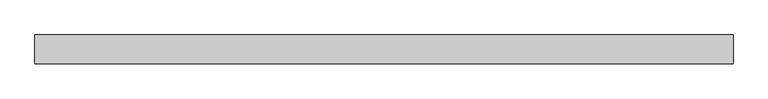
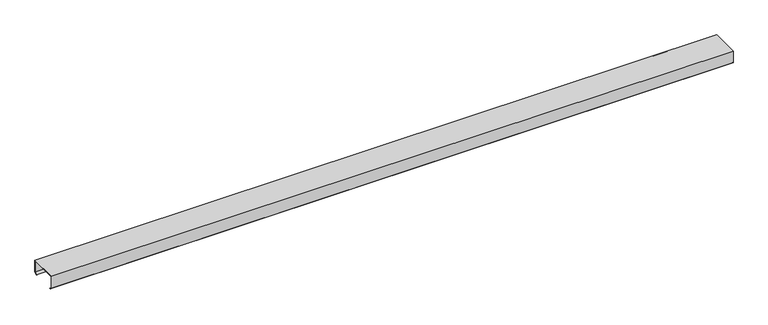
"""IFC4 building model written with IfcOpenShell, lengths in millimetres: proxy geometry, Generic Models 7:Generic Models 1:1:Generic Models 1:1 : Generic Models 7:Generic Models 1:337419:20 : Generic Models 7:Generic Models 1:1:Generic Models 1:1 : Generic Models 7:Generic Models 1:337419:306201."""

from ifc_helpers import new_model, si_unit, frame, origin, place, context, project, spatial, polyline, outline, extrude, source, transform, mapped, element, save


def generic_models_f52606a6(model_context):
    return source(origin(), model_context, "Body", "SweptSolid", [
        extrude(outline(polyline([(-578797.4913841, 4985.940625), (-578797.4913841, 4897.040625), (-578812.0845307, 4884.7955211), (-578813.870275, 4886.9236883), (-578800.2695091, 4898.336086), (-578800.2695091, 4983.1625), (-578997.9132591, 4983.1625), (-578997.9132591, 4898.336086), (-578984.3124931, 4886.9236883), (-578986.0982374, 4884.7955211), (-579000.6913841, 4897.040625), (-579000.6913841, 4985.940625), (-578797.4913841, 4985.940625)])), frame((574430.911724, 0.0, 0.0), z_axis=(1.0, 0.0, 0.0), x_axis=(0.0, 1.0, 0.0)), (0.0, 0.0, 1.0), 4876.7999999),
    ])


if __name__ == "__main__":
    model = new_model("IFC4")
    model_context = context("Model", 3, world=origin())
    ifc_project = project(units=[si_unit("LENGTHUNIT", "METRE", prefix="MILLI")], contexts=[model_context])
    site = spatial("IfcSite", under=ifc_project)
    building = spatial("IfcBuilding", under=site)
    placement = place(None, origin())
    generic_models_shape = generic_models_f52606a6(model_context)
    element("IfcBuildingElementProxy", 1, Name="Generic Models 7:Generic Models 1:1:Generic Models 1:1 : Generic Models 7:Generic Models 1:337419:20 : Generic Models 7:Generic Models 1:1:Generic Models 1:1 : Generic Models 7:Generic Models 1:337419:306201", ObjectType="Generic Models 7:Generic Models 1:1:Generic Models 1:1 : Generic Models 7:Generic Models 1:337419:20 : Generic Models 7:Generic Models 1:1:Generic Models 1:1 : Generic Models 7:Generic Models 1:337419:306201", at=placement, inside=building, context=model_context, shape_type="MappedRepresentation", body=[
        mapped(generic_models_shape, transform((0.0, 0.0, 0.0), x_axis=(1.0, 0.0, 0.0), y_axis=(0.0, 1.0, 0.0), z_axis=(0.0, 0.0, 1.0))),
    ])
    save(model, "model.ifc")

# Revit data of these elements
# Type "Generic Models 7:Generic Models 1:1:Generic Models 1:1 : Generic Models 7:Generic Models 1:337419:20 : Generic Models 7:Generic Models 1:1:Generic Models 1:1 : Generic Models 7:Generic Models 1:337419:306201"
#   NameOverride = "Generic Models 7:Generic Models 1:1:Generic Models 1:1 : Generic Models 7:Generic Models 1:337419:306201"
#   ObjectTypeOverride = "Generic Models 1:1 : Generic Models 7:Generic Models 1:337419"
#   Reference = "Generic Models 1"
#   Tag = "306201"
# Element 1 (IfcBuildingElementProxy, "Generic Models 7:Generic Models 1:1:Generic Models 1:1 : Generic Models 7:Generic Models 1:337419:20 : Generic Models 7:Generic Models 1:1:Generic Models 1:1 : Generic Models 7:Generic Models 1:337419:306201")
#   Materials on its faces: "'ZEE' SECTION (8.0x3.5Z - SEE STRUCT. DWGS)"
# Materials
#   "'ZEE' SECTION (8.0x3.5Z - SEE STRUCT. DWGS)": class "Unassigned", colour RGB 210 209 208, transparency 0, Keynote = "M05121300.02", Cost = 0
